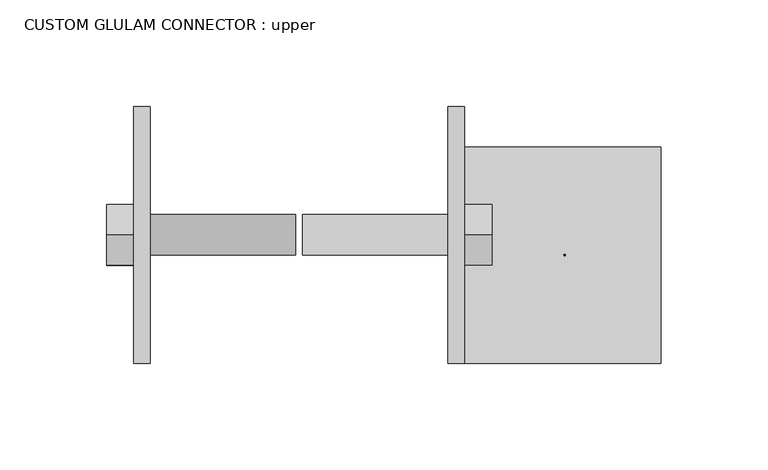
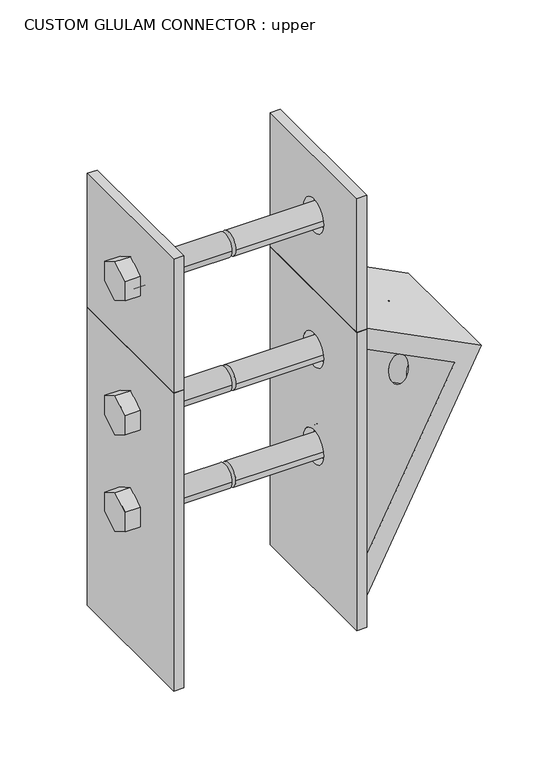
"""IFC4 building model written with IfcOpenShell, lengths in millimetres: fastener geometry, CUSTOM GLULAM CONNECTOR : upper."""

import ifcopenshell
import ifcopenshell.guid

model = None  # the IFC model being written
_history = None  # IfcOwnerHistory: only IFC2X3 demands one
_inside = {}  # id of a spatial element -> (the spatial element, [elements in it])
_under = {}  # id of a project, library or spatial element -> (it, [spatial elements below it])
_declared = {}  # id of a project -> (the project, [libraries it declares])
_typed = {}  # id of a type object -> (the type object, [elements of that type])
_made_of = {}  # id of a material, layer set ... -> (it, [elements and type objects made of it])


def new_model(schema):
    """Start an empty IFC model of exactly this schema.

    Asked for "IFC4X3", IfcOpenShell would pick the latest addendum, in which some entities
    have other attributes; the version numbers below select the first issue.
    IFC2X3 requires an IfcOwnerHistory on every rooted entity: one is made here for all.
    """
    global model, _history
    if schema == "IFC4X3":
        model = ifcopenshell.file(schema_version=(4, 3, 0, 0))
    else:
        model = ifcopenshell.file(schema=schema)
    _inside.clear()
    _under.clear()
    _declared.clear()
    _typed.clear()
    _made_of.clear()
    _history = None
    if model.schema == "IFC2X3":
        org = make("IfcOrganization", Name="unknown")
        user = make(
            "IfcPersonAndOrganization",
            ThePerson=make("IfcPerson", FamilyName="unknown"),
            TheOrganization=org,
        )
        app = make(
            "IfcApplication",
            ApplicationDeveloper=org,
            Version="unknown",
            ApplicationFullName="unknown",
            ApplicationIdentifier="unknown",
        )
        _history = make(
            "IfcOwnerHistory",
            OwningUser=user,
            OwningApplication=app,
            ChangeAction="ADDED",
            CreationDate=0,
        )
    return model


def make(cls, **values):
    """One entity of the class cls with the attributes given. An attribute that is None is left unset."""
    return model.create_entity(
        cls, **{name: value for name, value in values.items() if value is not None}
    )


def rooted(cls, **values):
    """An entity with a GlobalId (a new one), such as an element, a storey or a relation."""
    return make(cls, GlobalId=ifcopenshell.guid.new(), OwnerHistory=_history, **values)


def si_unit(unit_type, name, prefix=None):
    """IfcSIUnit, for example si_unit("LENGTHUNIT", "METRE", prefix="MILLI")."""
    return make("IfcSIUnit", UnitType=unit_type, Prefix=prefix, Name=name)


def assignment(units):
    """IfcUnitAssignment: the units of a project."""
    return None if units is None else make("IfcUnitAssignment", Units=units)


def point(xyz):
    """IfcCartesianPoint."""
    return None if xyz is None else make("IfcCartesianPoint", Coordinates=xyz)


def direction(xyz):
    """IfcDirection."""
    return None if xyz is None else make("IfcDirection", DirectionRatios=xyz)


def frame(location, z_axis=None, x_axis=None):
    """IfcAxis2Placement3D, a coordinate frame: its origin and axes. An axis left out is left unset."""
    return make(
        "IfcAxis2Placement3D",
        Location=point(location),
        Axis=direction(z_axis),
        RefDirection=direction(x_axis),
    )


def frame_2d(location, x_axis=None):
    """IfcAxis2Placement2D, a coordinate frame in the plane: its origin and x axis."""
    return make(
        "IfcAxis2Placement2D", Location=point(location), RefDirection=direction(x_axis)
    )


def origin():
    """The frame at (0, 0, 0) with its axes left unset."""
    return frame((0.0, 0.0, 0.0))


def place(relative_to, where):
    """IfcLocalPlacement: puts the frame where relative to a parent placement (None: the world)."""
    return make(
        "IfcLocalPlacement", PlacementRelTo=relative_to, RelativePlacement=where
    )


def context(
    kind, dimensions, precision=None, world=None, true_north=None, identifier=None
):
    """IfcGeometricRepresentationContext, for example the 3D "Model" context."""
    return make(
        "IfcGeometricRepresentationContext",
        ContextIdentifier=identifier,
        ContextType=kind,
        CoordinateSpaceDimension=dimensions,
        Precision=precision,
        WorldCoordinateSystem=world,
        TrueNorth=true_north,
    )


def project(units=None, contexts=None):
    """IfcProject with its units and contexts."""
    return rooted(
        "IfcProject",
        Name="project",
        RepresentationContexts=contexts,
        UnitsInContext=assignment(units),
    )


def spatial(cls, under=None, at=None, **own):
    """A site, building, storey or space (cls), placed at a placement, below another one or the project."""
    s = rooted(cls, ObjectPlacement=at, **own)
    if under is not None:
        _under.setdefault(under.id(), (under, []))[1].append(s)
    return s


def polyline(points):
    """IfcPolyline through the points."""
    return make("IfcPolyline", Points=[point(p) for p in points])


def circle_curve(where, radius):
    """IfcCircle in the frame where."""
    return make("IfcCircle", Position=where, Radius=radius)


def trimmed(basis, trim1, trim2, sense, master):
    """IfcTrimmedCurve: the piece of a basis curve between two trims."""
    return make(
        "IfcTrimmedCurve",
        BasisCurve=basis,
        Trim1=trim1,
        Trim2=trim2,
        SenseAgreement=sense,
        MasterRepresentation=master,
    )


def segment(curve, same_sense, transition):
    """IfcCompositeCurveSegment."""
    return make(
        "IfcCompositeCurveSegment",
        Transition=transition,
        SameSense=same_sense,
        ParentCurve=curve,
    )


def composite_curve(segments, self_intersect=None):
    """IfcCompositeCurve: segments joined end to end."""
    return make("IfcCompositeCurve", Segments=segments, SelfIntersect=self_intersect)


def outline(outer, holes=None, kind="AREA"):
    """IfcArbitraryClosedProfileDef: a profile drawn as a closed curve; with holes, ...WithVoids."""
    if holes is None:
        return make("IfcArbitraryClosedProfileDef", ProfileType=kind, OuterCurve=outer)
    return make(
        "IfcArbitraryProfileDefWithVoids",
        ProfileType=kind,
        OuterCurve=outer,
        InnerCurves=holes,
    )


def extrude(swept, where, along, depth):
    """IfcExtrudedAreaSolid: the profile swept, set in the frame where, extruded along a direction by depth."""
    return make(
        "IfcExtrudedAreaSolid",
        SweptArea=swept,
        Position=where,
        ExtrudedDirection=direction(along),
        Depth=depth,
    )


def shape(context_of_items, identifier, shape_type, items):
    """IfcShapeRepresentation: the items that make up one representation, for example the "Body"."""
    return make(
        "IfcShapeRepresentation",
        ContextOfItems=context_of_items,
        RepresentationIdentifier=identifier,
        RepresentationType=shape_type,
        Items=items,
    )


def source(mapping_origin, context_of_items, identifier, shape_type, items):
    """IfcRepresentationMap: a shape defined once, which mapped items show again and again."""
    return make(
        "IfcRepresentationMap",
        MappingOrigin=mapping_origin,
        MappedRepresentation=shape(context_of_items, identifier, shape_type, items),
    )


def transform(
    local_origin,
    x_axis=None,
    y_axis=None,
    z_axis=None,
    scale=None,
    scale2=None,
    scale3=None,
    uniform=True,
):
    """IfcCartesianTransformationOperator3D, or its non-uniform kind. x_axis, y_axis, z_axis: its Axis1, 2, 3."""
    if uniform:
        return make(
            "IfcCartesianTransformationOperator3D",
            Axis1=direction(x_axis),
            Axis2=direction(y_axis),
            LocalOrigin=point(local_origin),
            Scale=scale,
            Axis3=direction(z_axis),
        )
    return make(
        "IfcCartesianTransformationOperator3DnonUniform",
        Axis1=direction(x_axis),
        Axis2=direction(y_axis),
        LocalOrigin=point(local_origin),
        Scale=scale,
        Axis3=direction(z_axis),
        Scale2=scale2,
        Scale3=scale3,
    )


def mapped(mapping_source, mapping_target):
    """IfcMappedItem: shows the shape of a source again, moved by a transform."""
    return make(
        "IfcMappedItem", MappingSource=mapping_source, MappingTarget=mapping_target
    )


def made_of(thing, what):
    """Note that an element or type object is made of a material, layer set ...; save() writes the relation."""
    if what is not None:
        _made_of.setdefault(what.id(), (what, []))[1].append(thing)
    return thing


def element(
    cls,
    number,
    at=None,
    inside=None,
    cuts=None,
    type_object=None,
    material=None,
    context=None,
    identifier="Body",
    shape_type=None,
    held_by="IfcProductDefinitionShape",
    body=None,
    shapes=None,
    **own,
):
    """One element of the class cls, such as IfcWall. Its Tag is "e" and its number.

    at: its placement. inside: the storey or other place that contains it. cuts: it is an
    opening in that element (IfcRelVoidsElement). A single representation is given by context,
    identifier, shape_type and body (its items); several are given by shapes. held_by: the class
    of the entity that holds the representations. save() writes the other relations.
    """
    e = rooted(cls, Tag="e%d" % number, ObjectPlacement=at, **own)
    if body is not None:
        shapes = [shape(context, identifier, shape_type, body)]
    if shapes is not None:
        e.Representation = make(held_by, Representations=shapes)
    if inside is not None:
        _inside.setdefault(inside.id(), (inside, []))[1].append(e)
    if cuts is not None:
        rooted(
            "IfcRelVoidsElement", RelatingBuildingElement=cuts, RelatedOpeningElement=e
        )
    if type_object is not None:
        _typed.setdefault(type_object.id(), (type_object, []))[1].append(e)
    return made_of(e, material)


def aggregate(whole, parts):
    """IfcRelAggregates: a whole, such as a stair, and the parts it consists of."""
    return rooted("IfcRelAggregates", RelatingObject=whole, RelatedObjects=parts)


def save(model, path):
    """Write the relations noted so far, then the file.

    IfcRelAggregates (storeys below a building ...), IfcRelContainedInSpatialStructure (elements
    in a storey), IfcRelDefinesByType, IfcRelAssociatesMaterial and IfcRelDeclares: one each for
    every whole, place, type object, material and project.
    """
    for whole, parts in _under.values():
        aggregate(whole, parts)
    for where, things in _inside.values():
        rooted(
            "IfcRelContainedInSpatialStructure",
            RelatedElements=things,
            RelatingStructure=where,
        )
    for kind, things in _typed.values():
        rooted("IfcRelDefinesByType", RelatedObjects=things, RelatingType=kind)
    for what, things in _made_of.values():
        rooted("IfcRelAssociatesMaterial", RelatedObjects=things, RelatingMaterial=what)
    for by, libraries in _declared.values():
        rooted("IfcRelDeclares", RelatingContext=by, RelatedDefinitions=libraries)
    model.write(path)


def plane_surface(at):
    """IfcPlane: the flat surface through the origin of the frame at, square to its z axis."""
    return make("IfcPlane", Position=at)


def revolved_surface(curve, axis_point, axis_direction):
    """IfcSurfaceOfRevolution: the curve turned about the line through axis_point along axis_direction."""
    return make(
        "IfcSurfaceOfRevolution",
        SweptCurve=make("IfcArbitraryOpenProfileDef", ProfileType="CURVE", Curve=curve),
        AxisPosition=make("IfcAxis1Placement", Location=point(axis_point), Axis=direction(axis_direction)),
    )


def advanced_brep(points, edges, surfaces, faces):
    """IfcAdvancedBrep: a solid bounded by faces that lie on surfaces and meet in shared edges.

    An edge is (start, end): straight between two places in points (the first is 0);
    or (start, end, curve); or (start, end, curve, False) where it runs against its curve.
    A face is (place in surfaces, loops), or (place, loops, False) where it looks against
    its surface's normal. A loop lists edges by number (the first is 1), with a minus sign
    where the edge is run from its end to its start. The first loop is the outer one.
    """
    corners = [point(p) for p in points]
    vertices = [make("IfcVertexPoint", VertexGeometry=c) for c in corners]
    made = []
    for start, end, *more in edges:
        made.append(
            make(
                "IfcEdgeCurve",
                EdgeStart=vertices[start],
                EdgeEnd=vertices[end],
                EdgeGeometry=more[0] if more else make("IfcPolyline", Points=[corners[start], corners[end]]),
                SameSense=more[1] if len(more) > 1 else True,
            )
        )
    hull = []
    for where, loops, *sense in faces:
        bounds = []
        for j, loop in enumerate(loops):
            ring = [make("IfcOrientedEdge", EdgeElement=made[abs(k) - 1], Orientation=k > 0) for k in loop]
            bounds.append(
                make(
                    "IfcFaceOuterBound" if j == 0 else "IfcFaceBound",
                    Bound=make("IfcEdgeLoop", EdgeList=ring),
                    Orientation=True,
                )
            )
        hull.append(make("IfcAdvancedFace", Bounds=bounds, FaceSurface=surfaces[where], SameSense=sense[0] if sense else True))
    return make("IfcAdvancedBrep", Outer=make("IfcClosedShell", CfsFaces=hull))


def custom_glulam_connector_upper_734575cc(model_context):
    return source(origin(), model_context, "Body", "SolidModel", [
        advanced_brep(
        [(-77.7875, 60.325, 261.9375), (-77.7875, -52.3875, 261.9375), (-77.7875, -60.325, 261.9375), (-69.85, -60.325, 261.9375), (-69.85, 60.325, 261.9375), (-69.85, -60.325, 7.9375), (-69.85, 60.325, 7.9375), (-69.85, 13.890625, 211.1375), (-69.85, -13.890625, 211.1375), (-69.85, 13.890625, 128.5875), (-69.85, -13.890625, 128.5875), (-77.7875, 13.890625, 128.5875), (-77.7875, -13.890625, 128.5875), (-77.7875, 60.325, 7.9375), (-77.7875, -52.3875, 7.9375), (-77.7875, -60.325, 7.9375), (-77.7875, -13.890625, 211.1375), (-77.7875, 13.890625, 211.1375)],
        [
            (0, 1),
            (1, 2),
            (2, 3),
            (3, 4),
            (4, 0),
            (3, 5),
            (5, 6),
            (6, 4),
            (7, 8, circle_curve(frame((-69.85, 0.0, 211.1375), z_axis=(-1.0, 0.0, 0.0), x_axis=(0.0, -1.0, 0.0)), 13.890625)),
            (8, 7, circle_curve(frame((-69.85, 0.0, 211.1375), z_axis=(-1.0, 0.0, 0.0), x_axis=(0.0, -1.0, 0.0)), 13.890625)),
            (9, 10, circle_curve(frame((-69.85, 0.0, 128.5875), z_axis=(-1.0, 0.0, 0.0), x_axis=(0.0, -1.0, 0.0)), 13.890625)),
            (10, 9, circle_curve(frame((-69.85, 0.0, 128.5875), z_axis=(-1.0, 0.0, 0.0), x_axis=(0.0, -1.0, 0.0)), 13.890625)),
            (11, 9),
            (10, 12),
            (12, 11, circle_curve(frame((-77.7875, 0.0, 128.5875), z_axis=(-1.0, 0.0, 0.0), x_axis=(0.0, -1.0, 0.0)), 13.890625)),
            (0, 13),
            (13, 14),
            (14, 15),
            (15, 2),
            (16, 17, circle_curve(frame((-77.7875, 0.0, 211.1375), z_axis=(1.0, 0.0, 0.0), x_axis=(0.0, -1.0, 0.0)), 13.890625)),
            (17, 16, circle_curve(frame((-77.7875, 0.0, 211.1375), z_axis=(1.0, 0.0, 0.0), x_axis=(0.0, -1.0, 0.0)), 13.890625)),
            (12, 11, circle_curve(frame((-77.7875, 0.0, 128.5875), z_axis=(1.0, 0.0, 0.0), x_axis=(0.0, -1.0, 0.0)), 13.890625)),
            (6, 13),
            (15, 5),
            (7, 17),
            (16, 8),
        ],
        [
            plane_surface(frame((-77.7875, -60.325, 261.9375), z_axis=(0.0, 0.0, 1.0), x_axis=(1.0, 0.0, 0.0))),
            plane_surface(frame((-69.85, 60.325, 261.9375), z_axis=(1.0, 0.0, 0.0), x_axis=(0.0, -1.0, 0.0))),
            revolved_surface(polyline([(-77.7875, -13.890625, 128.5875), (-69.85, -13.890625, 128.5875)]), (-69.85, 0.0, 128.5875), (-1.0, 0.0, 0.0)),
            plane_surface(frame((-77.7875, 60.325, 261.9375), z_axis=(-1.0, 0.0, 0.0), x_axis=(0.0, 1.0, 0.0))),
            plane_surface(frame((-77.7875, 60.325, 261.9375), z_axis=(0.0, 1.0, 0.0), x_axis=(1.0, 0.0, 0.0))),
            plane_surface(frame((-77.7875, -60.325, 7.9375), z_axis=(0.0, -1.0, 0.0), x_axis=(1.0, 0.0, 0.0))),
            revolved_surface(polyline([(-77.7875, -13.890625, 211.1375), (-69.85, -13.890625, 211.1375)]), (-69.85, 0.0, 211.1375), (-1.0, 0.0, 0.0)),
            plane_surface(frame((-77.7875, 60.325, 7.9375), z_axis=(0.0, 0.0, -1.0), x_axis=(1.0, 0.0, 0.0))),
        ],
        [
            (0, [[1, 2, 3, 4, 5]]),
            (1, [[6, 7, 8, -4], [9, 10], [11, 12]]),
            (2, [[13, -12, 14, 15]]),
            (3, [[-2, -1, 16, 17, 18, 19], [20, 21], [22, -15]]),
            (4, [[-16, -5, -8, 23]]),
            (5, [[-19, 24, -6, -3]]),
            (6, [[25, -20, 26, -9]]),
            (6, [[-25, -10, -26, -21]]),
            (2, [[-13, -22, -14, -11]]),
            (7, [[-18, -17, -23, -7, -24]]),
        ],
    ),
        extrude(outline(polyline([(14.2875, 219.386392), (14.2875, 202.888608), (0.0, 194.6397161), (-14.2875, 202.888608), (-14.2875, 219.386392), (0.0, 227.6352839), (14.2875, 219.386392)])), frame((-90.4875, 0.0, 0.0), z_axis=(1.0, 0.0, 0.0), x_axis=(0.0, 1.0, 0.0)), (0.0, 0.0, 1.0), 12.7),
        extrude(outline(composite_curve([segment(trimmed(circle_curve(frame_2d((0.0, 211.1375)), 9.525), [point((9.525, 211.1375))], [point((-9.525, 211.1375))], False, "CARTESIAN"), True, "CONTINUOUS"), segment(trimmed(circle_curve(frame_2d((0.0, 211.1375)), 9.525), [point((-9.525, 211.1375))], [point((9.525, 211.1375))], False, "CARTESIAN"), True, "CONTINUOUS")], self_intersect=False)), frame((-77.7875, 0.0, 0.0), z_axis=(1.0, 0.0, 0.0), x_axis=(0.0, 1.0, 0.0)), (0.0, 0.0, 1.0), 76.2),
        extrude(outline(polyline([(14.2875, 136.836392), (14.2875, 120.338608), (0.0, 112.0897161), (-14.2875, 120.338608), (-14.2875, 136.836392), (0.0, 145.0852839), (14.2875, 136.836392)])), frame((-90.4875, 0.0, 0.0), z_axis=(1.0, 0.0, 0.0), x_axis=(0.0, 1.0, 0.0)), (0.0, 0.0, 1.0), 12.7),
        extrude(outline(composite_curve([segment(trimmed(circle_curve(frame_2d((0.0, 128.5875)), 9.525), [point((9.525, 128.5875))], [point((-9.525, 128.5875))], False, "CARTESIAN"), True, "CONTINUOUS"), segment(trimmed(circle_curve(frame_2d((0.0, 128.5875)), 9.525), [point((-9.525, 128.5875))], [point((9.525, 128.5875))], False, "CARTESIAN"), True, "CONTINUOUS")], self_intersect=False)), frame((-77.7875, 0.0, 0.0), z_axis=(1.0, 0.0, 0.0), x_axis=(0.0, 1.0, 0.0)), (0.0, 0.0, 1.0), 76.2),
        extrude(outline(polyline([(14.2875, 219.386392), (14.2875, 202.888608), (0.0, 194.6397161), (-14.2875, 202.888608), (-14.2875, 219.386392), (0.0, 227.6352839), (14.2875, 219.386392)])), frame((-90.4875, 0.0, 0.0), z_axis=(1.0, 0.0, 0.0), x_axis=(0.0, 1.0, 0.0)), (0.0, 0.0, 1.0), 12.7),
        extrude(outline(composite_curve([segment(trimmed(circle_curve(frame_2d((0.0, 211.1375)), 9.525), [point((9.525, 211.1375))], [point((-9.525, 211.1375))], False, "CARTESIAN"), True, "CONTINUOUS"), segment(trimmed(circle_curve(frame_2d((0.0, 211.1375)), 9.525), [point((-9.525, 211.1375))], [point((9.525, 211.1375))], False, "CARTESIAN"), True, "CONTINUOUS")], self_intersect=False)), frame((-77.7875, 0.0, 0.0), z_axis=(1.0, 0.0, 0.0), x_axis=(0.0, 1.0, 0.0)), (0.0, 0.0, 1.0), 76.2),
        advanced_brep(
        [(77.7875, 60.325, 261.9375), (69.85, 60.325, 261.9375), (69.85, -60.325, 261.9375), (77.7875, -60.325, 261.9375), (77.7875, -52.3875, 261.9375), (69.85, 60.325, 7.9375), (69.85, -60.325, 7.9375), (69.85, 13.890625, 211.1375), (69.85, -13.890625, 211.1375), (69.85, 13.890625, 128.5875), (69.85, -13.890625, 128.5875), (77.7875, 13.890625, 128.5875), (77.7875, -13.890625, 128.5875), (77.7875, -60.325, 7.9375), (77.7875, -52.3875, 7.9375), (77.7875, 60.325, 7.9375), (77.7875, -13.890625, 211.1375), (77.7875, 13.890625, 211.1375)],
        [
            (0, 1),
            (1, 2),
            (2, 3),
            (3, 4),
            (4, 0),
            (1, 5),
            (5, 6),
            (6, 2),
            (7, 8, circle_curve(frame((69.85, 0.0, 211.1375), z_axis=(1.0, 0.0, 0.0), x_axis=(0.0, -1.0, 0.0)), 13.890625)),
            (8, 7, circle_curve(frame((69.85, 0.0, 211.1375), z_axis=(1.0, 0.0, 0.0), x_axis=(0.0, -1.0, 0.0)), 13.890625)),
            (9, 10, circle_curve(frame((69.85, 0.0, 128.5875), z_axis=(1.0, 0.0, 0.0), x_axis=(0.0, -1.0, 0.0)), 13.890625)),
            (10, 9, circle_curve(frame((69.85, 0.0, 128.5875), z_axis=(1.0, 0.0, 0.0), x_axis=(0.0, -1.0, 0.0)), 13.890625)),
            (11, 12, circle_curve(frame((77.7875, 0.0, 128.5875), z_axis=(1.0, 0.0, 0.0), x_axis=(0.0, -1.0, 0.0)), 13.890625)),
            (12, 10),
            (9, 11),
            (3, 13),
            (13, 14),
            (14, 15),
            (15, 0),
            (16, 17, circle_curve(frame((77.7875, 0.0, 211.1375), z_axis=(-1.0, 0.0, 0.0), x_axis=(0.0, -1.0, 0.0)), 13.890625)),
            (17, 16, circle_curve(frame((77.7875, 0.0, 211.1375), z_axis=(-1.0, 0.0, 0.0), x_axis=(0.0, -1.0, 0.0)), 13.890625)),
            (11, 12, circle_curve(frame((77.7875, 0.0, 128.5875), z_axis=(-1.0, 0.0, 0.0), x_axis=(0.0, -1.0, 0.0)), 13.890625)),
            (15, 5),
            (6, 13),
            (8, 16),
            (17, 7),
        ],
        [
            plane_surface(frame((77.7875, -60.325, 261.9375), z_axis=(0.0, 0.0, 1.0), x_axis=(-1.0, 0.0, 0.0))),
            plane_surface(frame((69.85, 60.325, 261.9375), z_axis=(-1.0, 0.0, 0.0), x_axis=(0.0, -1.0, 0.0))),
            revolved_surface(polyline([(77.7875, -13.890625, 128.5875), (69.85, -13.890625, 128.5875)]), (69.85, 0.0, 128.5875), (1.0, 0.0, 0.0)),
            plane_surface(frame((77.7875, 60.325, 261.9375), z_axis=(1.0, 0.0, 0.0), x_axis=(0.0, 1.0, 0.0))),
            plane_surface(frame((77.7875, 60.325, 261.9375), z_axis=(0.0, 1.0, 0.0), x_axis=(-1.0, 0.0, 0.0))),
            plane_surface(frame((77.7875, -60.325, 7.9375), z_axis=(0.0, -1.0, 0.0), x_axis=(-1.0, 0.0, 0.0))),
            revolved_surface(polyline([(77.7875, -13.890625, 211.1375), (69.85, -13.890625, 211.1375)]), (69.85, 0.0, 211.1375), (1.0, 0.0, 0.0)),
            plane_surface(frame((77.7875, 60.325, 7.9375), z_axis=(0.0, 0.0, -1.0), x_axis=(-1.0, 0.0, 0.0))),
        ],
        [
            (0, [[1, 2, 3, 4, 5]]),
            (1, [[-2, 6, 7, 8], [9, 10], [11, 12]]),
            (2, [[13, 14, -11, 15]]),
            (3, [[16, 17, 18, 19, -5, -4], [20, 21], [-13, 22]]),
            (4, [[23, -6, -1, -19]]),
            (5, [[-3, -8, 24, -16]]),
            (6, [[-10, 25, -21, 26]]),
            (6, [[-20, -25, -9, -26]]),
            (2, [[-12, -14, -22, -15]]),
            (7, [[-24, -7, -23, -18, -17]]),
        ],
    ),
        extrude(outline(polyline([(14.2875, 219.386392), (14.2875, 202.888608), (0.0, 194.6397161), (-14.2875, 202.888608), (-14.2875, 219.386392), (0.0, 227.6352839), (14.2875, 219.386392)])), frame((77.7875, 0.0, 0.0), z_axis=(1.0, 0.0, 0.0), x_axis=(0.0, 1.0, 0.0)), (0.0, 0.0, 1.0), 12.7),
        extrude(outline(composite_curve([segment(trimmed(circle_curve(frame_2d((0.0, 211.1375)), 9.525), [point((9.525, 211.1375))], [point((-9.525, 211.1375))], False, "CARTESIAN"), True, "CONTINUOUS"), segment(trimmed(circle_curve(frame_2d((0.0, 211.1375)), 9.525), [point((-9.525, 211.1375))], [point((9.525, 211.1375))], False, "CARTESIAN"), True, "CONTINUOUS")], self_intersect=False)), frame((1.5875, 0.0, 0.0), z_axis=(1.0, 0.0, 0.0), x_axis=(0.0, 1.0, 0.0)), (0.0, 0.0, 1.0), 76.2),
        extrude(outline(polyline([(14.2875, 136.836392), (14.2875, 120.338608), (0.0, 112.0897161), (-14.2875, 120.338608), (-14.2875, 136.836392), (0.0, 145.0852839), (14.2875, 136.836392)])), frame((77.7875, 0.0, 0.0), z_axis=(1.0, 0.0, 0.0), x_axis=(0.0, 1.0, 0.0)), (0.0, 0.0, 1.0), 12.7),
        extrude(outline(composite_curve([segment(trimmed(circle_curve(frame_2d((0.0, 128.5875)), 9.525), [point((9.525, 128.5875))], [point((-9.525, 128.5875))], False, "CARTESIAN"), True, "CONTINUOUS"), segment(trimmed(circle_curve(frame_2d((0.0, 128.5875)), 9.525), [point((-9.525, 128.5875))], [point((9.525, 128.5875))], False, "CARTESIAN"), True, "CONTINUOUS")], self_intersect=False)), frame((1.5875, 0.0, 0.0), z_axis=(1.0, 0.0, 0.0), x_axis=(0.0, 1.0, 0.0)), (0.0, 0.0, 1.0), 76.2),
        extrude(outline(polyline([(14.2875, 219.386392), (14.2875, 202.888608), (0.0, 194.6397161), (-14.2875, 202.888608), (-14.2875, 219.386392), (0.0, 227.6352839), (14.2875, 219.386392)])), frame((77.7875, 0.0, 0.0), z_axis=(1.0, 0.0, 0.0), x_axis=(0.0, 1.0, 0.0)), (0.0, 0.0, 1.0), 12.7),
        extrude(outline(composite_curve([segment(trimmed(circle_curve(frame_2d((0.0, 211.1375)), 9.525), [point((9.525, 211.1375))], [point((-9.525, 211.1375))], False, "CARTESIAN"), True, "CONTINUOUS"), segment(trimmed(circle_curve(frame_2d((0.0, 211.1375)), 9.525), [point((-9.525, 211.1375))], [point((9.525, 211.1375))], False, "CARTESIAN"), True, "CONTINUOUS")], self_intersect=False)), frame((1.5875, 0.0, 0.0), z_axis=(1.0, 0.0, 0.0), x_axis=(0.0, 1.0, 0.0)), (0.0, 0.0, 1.0), 76.2),
        advanced_brep(
        [(-77.7875, 13.890625, 325.4375), (-69.85, 13.890625, 325.4375), (-69.85, -13.890625, 325.4375), (-77.7875, -13.890625, 325.4375), (-77.7875, -60.325, 376.2375), (-77.7875, 60.325, 376.2375), (-77.7875, 60.325, 261.9375), (-77.7875, 52.3875, 261.9375), (-77.7875, -60.325, 261.9375), (-69.85, 60.325, 376.2375), (-69.85, 60.325, 261.9375), (-69.85, -60.325, 261.9375), (-69.85, -60.325, 376.2375)],
        [
            (0, 1),
            (1, 2, circle_curve(frame((-69.85, 0.0, 325.4375), z_axis=(1.0, 0.0, 0.0), x_axis=(0.0, -1.0, 0.0)), 13.890625)),
            (2, 3),
            (3, 0, circle_curve(frame((-77.7875, 0.0, 325.4375), z_axis=(-1.0, 0.0, 0.0), x_axis=(0.0, -1.0, 0.0)), 13.890625)),
            (4, 5),
            (5, 6),
            (6, 7),
            (7, 8),
            (8, 4),
            (3, 0, circle_curve(frame((-77.7875, 0.0, 325.4375), z_axis=(1.0, 0.0, 0.0), x_axis=(0.0, -1.0, 0.0)), 13.890625)),
            (5, 9),
            (9, 10),
            (10, 6),
            (8, 11),
            (11, 12),
            (12, 4),
            (2, 1, circle_curve(frame((-69.85, 0.0, 325.4375), z_axis=(1.0, 0.0, 0.0), x_axis=(0.0, -1.0, 0.0)), 13.890625)),
            (12, 9),
            (11, 10),
        ],
        [
            revolved_surface(polyline([(-77.7875, -13.890625, 325.4375), (-69.85, -13.890625, 325.4375)]), (-69.85, 0.0, 325.4375), (-1.0, 0.0, 0.0)),
            plane_surface(frame((-77.7875, 60.325, 376.2375), z_axis=(-1.0, 0.0, 0.0), x_axis=(0.0, 1.0, 0.0))),
            plane_surface(frame((-77.7875, 60.325, 376.2375), z_axis=(0.0, 1.0, 0.0), x_axis=(1.0, 0.0, 0.0))),
            plane_surface(frame((-77.7875, -60.325, 261.9375), z_axis=(0.0, -1.0, 0.0), x_axis=(1.0, 0.0, 0.0))),
            plane_surface(frame((-77.7875, -60.325, 376.2375), z_axis=(0.0, 0.0, 1.0), x_axis=(1.0, 0.0, 0.0))),
            plane_surface(frame((-69.85, 60.325, 376.2375), z_axis=(1.0, 0.0, 0.0), x_axis=(0.0, -1.0, 0.0))),
            plane_surface(frame((-77.7875, 60.325, 261.9375), z_axis=(0.0, 0.0, -1.0), x_axis=(1.0, 0.0, 0.0))),
        ],
        [
            (0, [[1, 2, 3, 4]]),
            (1, [[5, 6, 7, 8, 9], [10, -4]]),
            (2, [[-6, 11, 12, 13]]),
            (3, [[-9, 14, 15, 16]]),
            (0, [[-1, -10, -3, 17]]),
            (4, [[-5, -16, 18, -11]]),
            (5, [[-15, 19, -12, -18], [-17, -2]]),
            (6, [[-8, -7, -13, -19, -14]]),
        ],
    ),
        extrude(outline(polyline([(14.2875, 333.686392), (14.2875, 317.188608), (0.0, 308.9397161), (-14.2875, 317.188608), (-14.2875, 333.686392), (0.0, 341.9352839), (14.2875, 333.686392)])), frame((-90.4875, 0.0, 0.0), z_axis=(1.0, 0.0, 0.0), x_axis=(0.0, 1.0, 0.0)), (0.0, 0.0, 1.0), 12.7),
        extrude(outline(composite_curve([segment(trimmed(circle_curve(frame_2d((0.0, 325.4375)), 9.525), [point((9.525, 325.4375))], [point((-9.525, 325.4375))], False, "CARTESIAN"), True, "CONTINUOUS"), segment(trimmed(circle_curve(frame_2d((0.0, 325.4375)), 9.525), [point((-9.525, 325.4375))], [point((9.525, 325.4375))], False, "CARTESIAN"), True, "CONTINUOUS")], self_intersect=False)), frame((-77.7875, 0.0, 0.0), z_axis=(1.0, 0.0, 0.0), x_axis=(0.0, 1.0, 0.0)), (0.0, 0.0, 1.0), 76.2),
        advanced_brep(
        [(77.7875, 13.890625, 325.4375), (77.7875, -13.890625, 325.4375), (69.85, -13.890625, 325.4375), (69.85, 13.890625, 325.4375), (77.7875, -60.325, 376.2375), (77.7875, -60.325, 261.9375), (77.7875, 52.3875, 261.9375), (77.7875, 60.325, 261.9375), (77.7875, 60.325, 376.2375), (69.85, 60.325, 261.9375), (69.85, 60.325, 376.2375), (69.85, -60.325, 376.2375), (69.85, -60.325, 261.9375)],
        [
            (0, 1, circle_curve(frame((77.7875, 0.0, 325.4375), z_axis=(1.0, 0.0, 0.0), x_axis=(0.0, -1.0, 0.0)), 13.890625)),
            (1, 2),
            (2, 3, circle_curve(frame((69.85, 0.0, 325.4375), z_axis=(-1.0, 0.0, 0.0), x_axis=(0.0, -1.0, 0.0)), 13.890625)),
            (3, 0),
            (4, 5),
            (5, 6),
            (6, 7),
            (7, 8),
            (8, 4),
            (0, 1, circle_curve(frame((77.7875, 0.0, 325.4375), z_axis=(-1.0, 0.0, 0.0), x_axis=(0.0, -1.0, 0.0)), 13.890625)),
            (7, 9),
            (9, 10),
            (10, 8),
            (4, 11),
            (11, 12),
            (12, 5),
            (3, 2, circle_curve(frame((69.85, 0.0, 325.4375), z_axis=(-1.0, 0.0, 0.0), x_axis=(0.0, -1.0, 0.0)), 13.890625)),
            (10, 11),
            (9, 12),
        ],
        [
            revolved_surface(polyline([(77.7875, -13.890625, 325.4375), (69.85, -13.890625, 325.4375)]), (69.85, 0.0, 325.4375), (1.0, 0.0, 0.0)),
            plane_surface(frame((77.7875, 60.325, 376.2375), z_axis=(1.0, 0.0, 0.0), x_axis=(0.0, 1.0, 0.0))),
            plane_surface(frame((77.7875, 60.325, 376.2375), z_axis=(0.0, 1.0, 0.0), x_axis=(-1.0, 0.0, 0.0))),
            plane_surface(frame((77.7875, -60.325, 261.9375), z_axis=(0.0, -1.0, 0.0), x_axis=(-1.0, 0.0, 0.0))),
            plane_surface(frame((77.7875, -60.325, 376.2375), z_axis=(0.0, 0.0, 1.0), x_axis=(-1.0, 0.0, 0.0))),
            plane_surface(frame((69.85, 60.325, 376.2375), z_axis=(-1.0, 0.0, 0.0), x_axis=(0.0, -1.0, 0.0))),
            plane_surface(frame((77.7875, 60.325, 261.9375), z_axis=(0.0, 0.0, -1.0), x_axis=(-1.0, 0.0, 0.0))),
        ],
        [
            (0, [[1, 2, 3, 4]]),
            (1, [[5, 6, 7, 8, 9], [-1, 10]]),
            (2, [[11, 12, 13, -8]]),
            (3, [[14, 15, 16, -5]]),
            (0, [[17, -2, -10, -4]]),
            (4, [[-13, 18, -14, -9]]),
            (5, [[-18, -12, 19, -15], [-3, -17]]),
            (6, [[-16, -19, -11, -7, -6]]),
        ],
    ),
        extrude(outline(polyline([(14.2875, 333.686392), (14.2875, 317.188608), (0.0, 308.9397161), (-14.2875, 317.188608), (-14.2875, 333.686392), (0.0, 341.9352839), (14.2875, 333.686392)])), frame((77.7875, 0.0, 0.0), z_axis=(1.0, 0.0, 0.0), x_axis=(0.0, 1.0, 0.0)), (0.0, 0.0, 1.0), 12.7),
        extrude(outline(composite_curve([segment(trimmed(circle_curve(frame_2d((0.0, 325.4375)), 9.525), [point((9.525, 325.4375))], [point((-9.525, 325.4375))], False, "CARTESIAN"), True, "CONTINUOUS"), segment(trimmed(circle_curve(frame_2d((0.0, 325.4375)), 9.525), [point((-9.525, 325.4375))], [point((9.525, 325.4375))], False, "CARTESIAN"), True, "CONTINUOUS")], self_intersect=False)), frame((1.5875, 0.0, 0.0), z_axis=(1.0, 0.0, 0.0), x_axis=(0.0, 1.0, 0.0)), (0.0, 0.0, 1.0), 76.2),
        advanced_brep(
        [(170.0383695, 41.275, 215.9775257), (77.7875, 41.275, 34.925), (77.7875, 41.275, 69.8926921), (148.6865418, 41.275, 209.0398963), (77.7875, 41.275, 245.1647625), (77.7875, 41.275, 262.9816915), (170.0383695, -60.325, 215.9775257), (77.7875, -60.325, 262.9816915), (77.7875, -60.325, 245.1647625), (148.6865418, -60.325, 209.0398963), (77.7875, -60.325, 69.8926921), (77.7875, -60.325, 34.925), (125.1288563, -9.525, 238.8600656), (124.4216199, -9.525, 239.2204206), (117.2145207, -9.525, 225.075692), (117.9217571, -9.525, 224.7153371), (137.6957155, -9.525, 187.4691853), (127.9661316, -9.525, 168.3738017), (142.1108602, -9.525, 161.1667025), (151.8404441, -9.525, 180.2620861)],
        [
            (0, 1),
            (1, 2),
            (2, 3),
            (3, 4),
            (4, 5),
            (5, 0),
            (6, 7),
            (7, 8),
            (8, 9),
            (9, 10),
            (10, 11),
            (11, 6),
            (5, 7),
            (6, 0),
            (12, 13, circle_curve(frame((124.7752381, -9.525, 239.0402431), z_axis=(-0.45399049973954897, 0.0, -0.8910065241883668), x_axis=(-0.8910065241883668, 0.0, 0.45399049973954897)), 0.396875)),
            (13, 12, circle_curve(frame((124.7752381, -9.525, 239.0402431), z_axis=(-0.45399049973954897, 0.0, -0.8910065241883668), x_axis=(-0.8910065241883668, 0.0, 0.45399049973954897)), 0.396875)),
            (4, 8),
            (3, 9),
            (14, 15, circle_curve(frame((117.5681389, -9.525, 224.8955145), z_axis=(0.45399049973954897, 0.0, 0.8910065241883668), x_axis=(-0.8910065241883668, 0.0, 0.45399049973954897)), 0.396875)),
            (15, 14, circle_curve(frame((117.5681389, -9.525, 224.8955145), z_axis=(0.45399049973954897, 0.0, 0.8910065241883668), x_axis=(-0.8910065241883668, 0.0, 0.45399049973954897)), 0.396875)),
            (2, 10),
            (16, 17, circle_curve(frame((132.8309236, -9.525, 177.9214935), z_axis=(0.8910065241883661, 0.0, -0.4539904997395502), x_axis=(0.4539904997395502, 0.0, 0.8910065241883661)), 10.715625)),
            (17, 16, circle_curve(frame((132.8309236, -9.525, 177.9214935), z_axis=(0.8910065241883661, 0.0, -0.4539904997395502), x_axis=(0.4539904997395502, 0.0, 0.8910065241883661)), 10.715625)),
            (1, 11),
            (18, 19, circle_curve(frame((146.9756522, -9.525, 170.7143943), z_axis=(-0.8910065241883661, 0.0, 0.4539904997395502), x_axis=(0.4539904997395502, 0.0, 0.8910065241883661)), 10.715625)),
            (19, 18, circle_curve(frame((146.9756522, -9.525, 170.7143943), z_axis=(-0.8910065241883661, 0.0, 0.4539904997395502), x_axis=(0.4539904997395502, 0.0, 0.8910065241883661)), 10.715625)),
            (13, 14),
            (15, 12),
            (19, 16),
            (17, 18),
        ],
        [
            plane_surface(frame((77.7875, 41.275, 262.9816915), z_axis=(0.0, 1.0, 0.0), x_axis=(-0.8910065241883668, 0.0, 0.45399049973954897))),
            plane_surface(frame((77.7875, -60.325, 262.9816915), z_axis=(0.0, -1.0, 0.0), x_axis=(0.8910065241883668, 0.0, -0.45399049973954897))),
            plane_surface(frame((170.0383695, 41.275, 215.9775257), z_axis=(0.45399049973954897, 0.0, 0.8910065241883668), x_axis=(0.0, -1.0, 0.0))),
            plane_surface(frame((77.7875, 41.275, 262.9816915), z_axis=(-1.0, 0.0, 0.0), x_axis=(0.0, -1.0, 0.0))),
            plane_surface(frame((77.7875, 41.275, 245.1647625), z_axis=(-0.4539904997395488, 0.0, -0.8910065241883668), x_axis=(0.0, -1.0, 0.0))),
            plane_surface(frame((148.6865418, 41.275, 209.0398963), z_axis=(-0.8910065241883659, 0.0, 0.45399049973955063), x_axis=(0.0, -1.0, 0.0))),
            plane_surface(frame((77.7875, 41.275, 69.8926921), z_axis=(-1.0, 0.0, 0.0), x_axis=(0.0, -1.0, 0.0))),
            plane_surface(frame((77.7875, 41.275, 34.925), z_axis=(0.8910065241883661, 0.0, -0.4539904997395502), x_axis=(0.0, -1.0, 0.0))),
            revolved_surface(polyline([(117.21452068738647, -9.525, 225.0756919787313), (124.42161989691586, -9.525, 239.22042060157148)]), (124.7752381, -9.525, 239.0402431), (-0.45399049973954897, 0.0, -0.8910065241883668)),
            revolved_surface(polyline([(137.69571550343758, -9.525, 187.4691853067466), (151.84044414877164, -9.525, 180.26208608575598)]), (146.9756522, -9.525, 170.7143943), (-0.8910065241883661, 0.0, 0.4539904997395502)),
        ],
        [
            (0, [[1, 2, 3, 4, 5, 6]]),
            (1, [[7, 8, 9, 10, 11, 12]]),
            (2, [[13, -7, 14, -6], [15, 16]]),
            (3, [[17, -8, -13, -5]]),
            (4, [[18, -9, -17, -4], [19, 20]]),
            (5, [[21, -10, -18, -3], [22, 23]]),
            (6, [[24, -11, -21, -2]]),
            (7, [[-14, -12, -24, -1], [25, 26]]),
            (8, [[-16, 27, -20, 28]]),
            (8, [[-19, -27, -15, -28]]),
            (9, [[-26, 29, -23, 30]]),
            (9, [[-22, -29, -25, -30]]),
        ],
    ),
    ])


if __name__ == "__main__":
    model = new_model("IFC4")
    model_context = context("Model", 3, world=origin())
    ifc_project = project(units=[si_unit("LENGTHUNIT", "METRE", prefix="MILLI")], contexts=[model_context])
    site = spatial("IfcSite", under=ifc_project)
    building = spatial("IfcBuilding", under=site)
    placement = place(None, origin())
    custom_glulam_connector_upper_shape = custom_glulam_connector_upper_734575cc(model_context)
    element("IfcFastener", 1, ObjectType="CUSTOM GLULAM CONNECTOR : upper", at=placement, inside=building, context=model_context, shape_type="MappedRepresentation", body=[
        mapped(custom_glulam_connector_upper_shape, transform((0.0, 0.0, 0.0), x_axis=(1.0, 0.0, 0.0), y_axis=(0.0, 1.0, 0.0), z_axis=(0.0, 0.0, 1.0))),
    ])
    save(model, "model.ifc")

# Revit data of these elements
# Type "CUSTOM GLULAM CONNECTOR : upper"
#   Width - Top = 0' - 5 1/2"
#   Top/Bottom Plate Thickness = 0' - 0 5/16"
#   Top/Bottom Plate - Width = 0' - 7 1/2"
#   Rod Radius = 0' - 0 3/8"
#   Rod Length [instance default] = 1' - 0"
#   Plate Thickness = 0' - 0 5/16"
#   Offset - Upper Plate 2 = 0' - 0"
#   Height of Plate = 0' - 10"
#   Width - Bottom = 0' - 5 1/2"
#   Plate Width = 0' - 4 3/4"
#   Bracket Width = 0' - 4"
#   Bracket Thickness = 0' - 0 5/8"
#   Bracket Offset in X = 0' - 3 1/16"
#   Bracket Offset in Y = 0' - 0"
#   Bracket Offset = 0' - 1 3/8"
#   Bracket Leg = 0' - 8"
#   Bracket Hole Radius - Up = 0' - 0 1/64"
#   Bracket Hole Radius - Down = 0' - 0 27/64"
#   Bracket Hole Offset = 0' - 2"
#   Beam Width = 0' - 7 3/8"
#   Angle 2 = 63.00°
#   Angle 1 = 153.00°
#   Top Plate Visible = no
#   Rod Visibility = no
#   Plate Visibility - Upper Right 2 = no
#   Plate Visibility - Upper Right 1 = yes
#   Plate Visibility - Upper Left 2 = no
#   Plate Visibility - Upper Left 1 = yes
#   Plate Visibility - Lower Right 2 = no
#   Plate Visibility - Lower Right 1 = yes
#   Plate Visibility - Lower Left 2 = no
#   Plate Visibility - Lower Left 1 = yes
#   Bracket Visibility = yes
#   Bottom Plate Visible = no
#   Upper Plates - 2 = element 1407874
#   Upper Plates - 1 = element 1407868
#   Lower Plates = element 1407872
#   Bracket Material = 5/8" STEEL ANGLE (HDG AFTER FABRICATION)
#   URL = ""
# Element 1 (IfcFastener, "CUSTOM GLULAM CONNECTOR : upper")
#   Materials on its faces: "3/4\" LAG BOLT (THRU BOLT IF PLATE ON OPP. SIDE OF STRUCT MEMBER)", "5/16\" STEEL PLATE (HDG AFTER FABRICATION)", "5/8\" STEEL ANGLE (HDG AFTER FABRICATION)"
# Materials
#   "5/8\" STEEL ANGLE (HDG AFTER FABRICATION)": class "Generic", colour RGB 195 195 195, transparency 0, Cost = 0
#   "3/4\" LAG BOLT (THRU BOLT IF PLATE ON OPP. SIDE OF STRUCT MEMBER)": class "Generic", colour RGB 120 120 120, transparency 0, Cost = 0
#   "5/16\" STEEL PLATE (HDG AFTER FABRICATION)": class "Generic", colour RGB 232 232 232, transparency 0, Cost = 0
